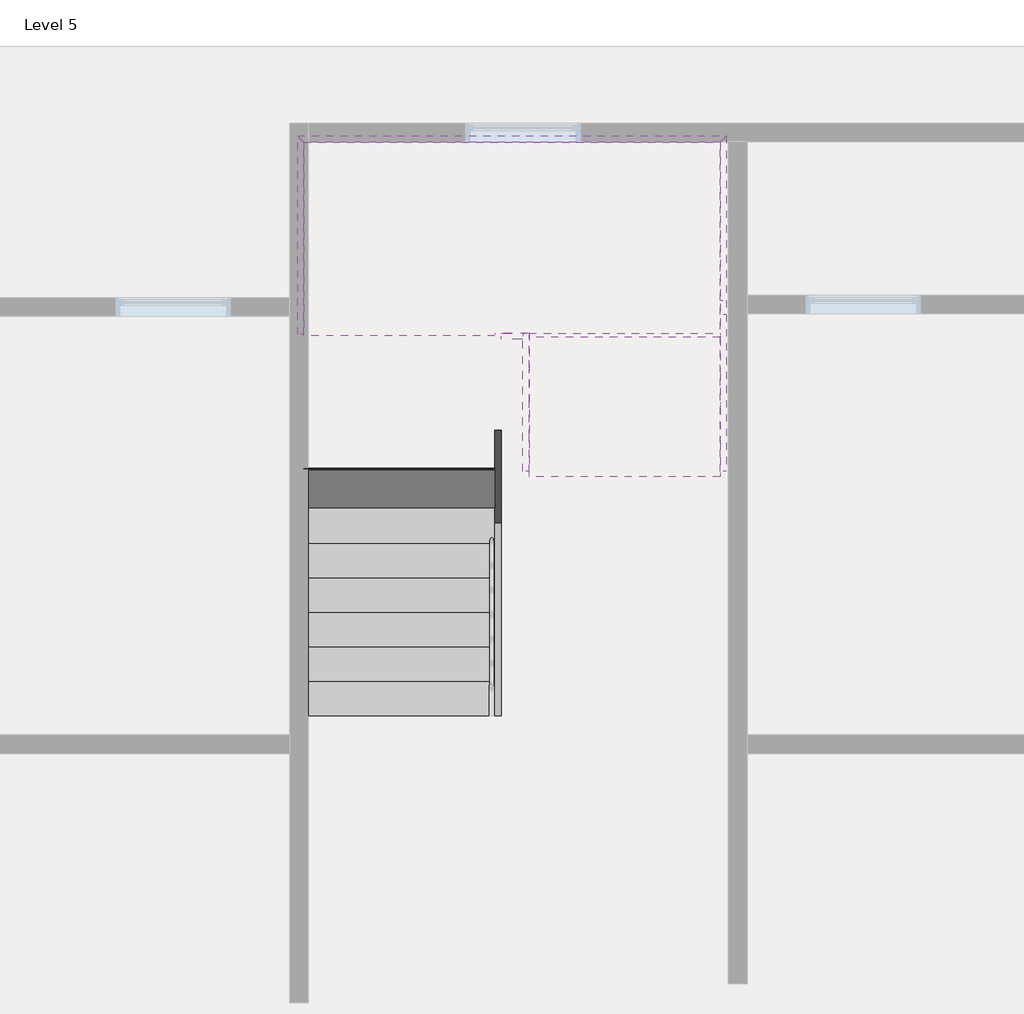
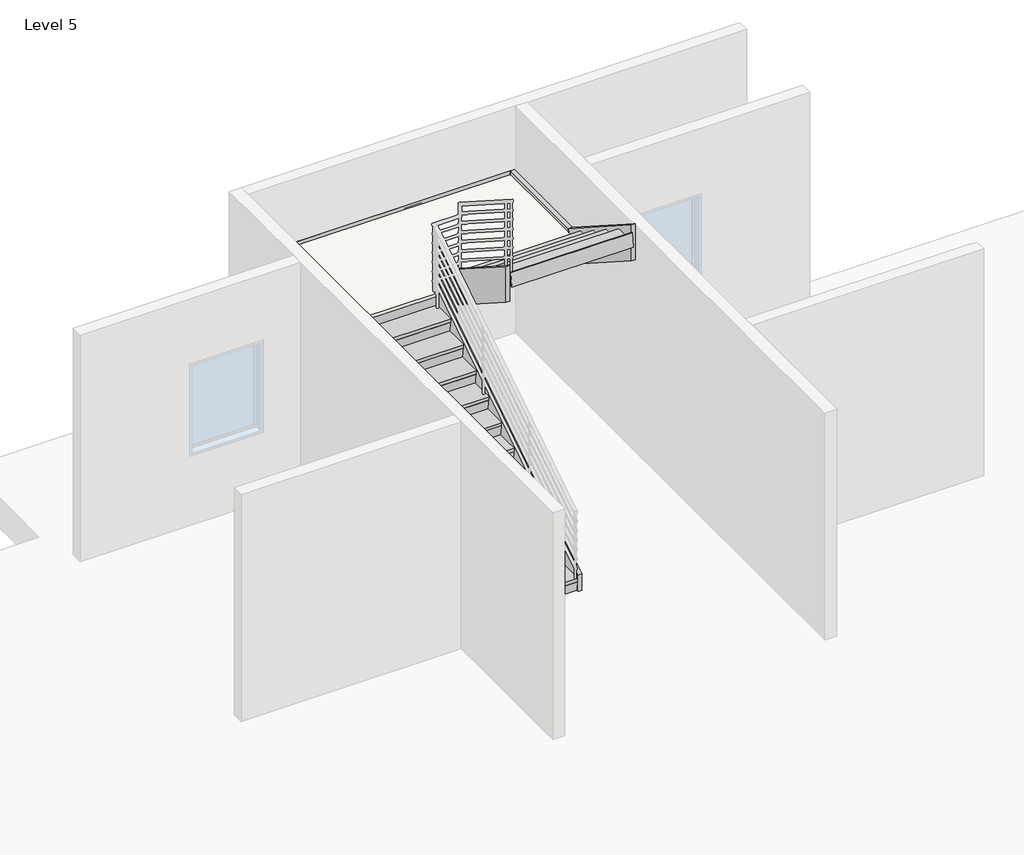
# One storey, part 7 of 7: 8 members, 2 stair flights, 1 slab.
"""IFC4 building model written with IfcOpenShell, lengths in millimetres."""

import ifcopenshell
import ifcopenshell.guid

model = None  # the IFC model being written
_history = None  # IfcOwnerHistory: only IFC2X3 demands one
_inside = {}  # id of a spatial element -> (the spatial element, [elements in it])
_under = {}  # id of a project, library or spatial element -> (it, [spatial elements below it])
_declared = {}  # id of a project -> (the project, [libraries it declares])
_typed = {}  # id of a type object -> (the type object, [elements of that type])
_made_of = {}  # id of a material, layer set ... -> (it, [elements and type objects made of it])


def new_model(schema):
    """Start an empty IFC model of exactly this schema.

    Asked for "IFC4X3", IfcOpenShell would pick the latest addendum, in which some entities
    have other attributes; the version numbers below select the first issue.
    IFC2X3 requires an IfcOwnerHistory on every rooted entity: one is made here for all.
    """
    global model, _history
    if schema == "IFC4X3":
        model = ifcopenshell.file(schema_version=(4, 3, 0, 0))
    else:
        model = ifcopenshell.file(schema=schema)
    _inside.clear()
    _under.clear()
    _declared.clear()
    _typed.clear()
    _made_of.clear()
    _history = None
    if model.schema == "IFC2X3":
        org = make("IfcOrganization", Name="unknown")
        user = make(
            "IfcPersonAndOrganization",
            ThePerson=make("IfcPerson", FamilyName="unknown"),
            TheOrganization=org,
        )
        app = make(
            "IfcApplication",
            ApplicationDeveloper=org,
            Version="unknown",
            ApplicationFullName="unknown",
            ApplicationIdentifier="unknown",
        )
        _history = make(
            "IfcOwnerHistory",
            OwningUser=user,
            OwningApplication=app,
            ChangeAction="ADDED",
            CreationDate=0,
        )
    return model


def make(cls, **values):
    """One entity of the class cls with the attributes given. An attribute that is None is left unset."""
    return model.create_entity(
        cls, **{name: value for name, value in values.items() if value is not None}
    )


def rooted(cls, **values):
    """An entity with a GlobalId (a new one), such as an element, a storey or a relation."""
    return make(cls, GlobalId=ifcopenshell.guid.new(), OwnerHistory=_history, **values)


def si_unit(unit_type, name, prefix=None):
    """IfcSIUnit, for example si_unit("LENGTHUNIT", "METRE", prefix="MILLI")."""
    return make("IfcSIUnit", UnitType=unit_type, Prefix=prefix, Name=name)


def assignment(units):
    """IfcUnitAssignment: the units of a project."""
    return None if units is None else make("IfcUnitAssignment", Units=units)


def point(xyz):
    """IfcCartesianPoint."""
    return None if xyz is None else make("IfcCartesianPoint", Coordinates=xyz)


def direction(xyz):
    """IfcDirection."""
    return None if xyz is None else make("IfcDirection", DirectionRatios=xyz)


def frame(location, z_axis=None, x_axis=None):
    """IfcAxis2Placement3D, a coordinate frame: its origin and axes. An axis left out is left unset."""
    return make(
        "IfcAxis2Placement3D",
        Location=point(location),
        Axis=direction(z_axis),
        RefDirection=direction(x_axis),
    )


def origin():
    """The frame at (0, 0, 0) with its axes left unset."""
    return frame((0.0, 0.0, 0.0))


def place(relative_to, where):
    """IfcLocalPlacement: puts the frame where relative to a parent placement (None: the world)."""
    return make(
        "IfcLocalPlacement", PlacementRelTo=relative_to, RelativePlacement=where
    )


def context(
    kind, dimensions, precision=None, world=None, true_north=None, identifier=None
):
    """IfcGeometricRepresentationContext, for example the 3D "Model" context."""
    return make(
        "IfcGeometricRepresentationContext",
        ContextIdentifier=identifier,
        ContextType=kind,
        CoordinateSpaceDimension=dimensions,
        Precision=precision,
        WorldCoordinateSystem=world,
        TrueNorth=true_north,
    )


def project(units=None, contexts=None):
    """IfcProject with its units and contexts."""
    return rooted(
        "IfcProject",
        Name="project",
        RepresentationContexts=contexts,
        UnitsInContext=assignment(units),
    )


def spatial(cls, under=None, at=None, **own):
    """A site, building, storey or space (cls), placed at a placement, below another one or the project."""
    s = rooted(cls, ObjectPlacement=at, **own)
    if under is not None:
        _under.setdefault(under.id(), (under, []))[1].append(s)
    return s


def polyline(points):
    """IfcPolyline through the points."""
    return make("IfcPolyline", Points=[point(p) for p in points])


def outline(outer, holes=None, kind="AREA"):
    """IfcArbitraryClosedProfileDef: a profile drawn as a closed curve; with holes, ...WithVoids."""
    if holes is None:
        return make("IfcArbitraryClosedProfileDef", ProfileType=kind, OuterCurve=outer)
    return make(
        "IfcArbitraryProfileDefWithVoids",
        ProfileType=kind,
        OuterCurve=outer,
        InnerCurves=holes,
    )


def extrude(swept, where, along, depth):
    """IfcExtrudedAreaSolid: the profile swept, set in the frame where, extruded along a direction by depth."""
    return make(
        "IfcExtrudedAreaSolid",
        SweptArea=swept,
        Position=where,
        ExtrudedDirection=direction(along),
        Depth=depth,
    )


def faces_of(points, faces, orient=None, outer=None):
    """IfcFace entities. A face is a list of loops; a loop is a list of indices into points, from 0.

    orient and outer hold one flag for each loop. By default every Orientation is true, the
    first loop of a face is its IfcFaceOuterBound and the others are IfcFaceBound.
    """
    made = []
    for i, loops in enumerate(faces):
        bounds = []
        for j, loop in enumerate(loops):
            is_outer = j == 0 if outer is None else outer[i][j]
            bounds.append(
                make(
                    "IfcFaceOuterBound" if is_outer else "IfcFaceBound",
                    Bound=make("IfcPolyLoop", Polygon=[points[k] for k in loop]),
                    Orientation=True if orient is None else orient[i][j],
                )
            )
        made.append(make("IfcFace", Bounds=bounds))
    return made


def faceted_brep(points, faces, orient=None, outer=None, voids=None):
    """IfcFacetedBrep: a solid bounded by flat faces; with voids (closed shells), ...WithVoids."""
    shared = [point(p) for p in points]
    hull = make("IfcClosedShell", CfsFaces=faces_of(shared, faces, orient, outer))
    if voids is None:
        return make("IfcFacetedBrep", Outer=hull)
    return make(
        "IfcFacetedBrepWithVoids",
        Outer=hull,
        Voids=[
            make(cls, CfsFaces=faces_of(shared, fs, o, b)) for cls, fs, o, b in voids
        ],
    )


def shape(context_of_items, identifier, shape_type, items):
    """IfcShapeRepresentation: the items that make up one representation, for example the "Body"."""
    return make(
        "IfcShapeRepresentation",
        ContextOfItems=context_of_items,
        RepresentationIdentifier=identifier,
        RepresentationType=shape_type,
        Items=items,
    )


def source(mapping_origin, context_of_items, identifier, shape_type, items):
    """IfcRepresentationMap: a shape defined once, which mapped items show again and again."""
    return make(
        "IfcRepresentationMap",
        MappingOrigin=mapping_origin,
        MappedRepresentation=shape(context_of_items, identifier, shape_type, items),
    )


def transform(
    local_origin,
    x_axis=None,
    y_axis=None,
    z_axis=None,
    scale=None,
    scale2=None,
    scale3=None,
    uniform=True,
):
    """IfcCartesianTransformationOperator3D, or its non-uniform kind. x_axis, y_axis, z_axis: its Axis1, 2, 3."""
    if uniform:
        return make(
            "IfcCartesianTransformationOperator3D",
            Axis1=direction(x_axis),
            Axis2=direction(y_axis),
            LocalOrigin=point(local_origin),
            Scale=scale,
            Axis3=direction(z_axis),
        )
    return make(
        "IfcCartesianTransformationOperator3DnonUniform",
        Axis1=direction(x_axis),
        Axis2=direction(y_axis),
        LocalOrigin=point(local_origin),
        Scale=scale,
        Axis3=direction(z_axis),
        Scale2=scale2,
        Scale3=scale3,
    )


def mapped(mapping_source, mapping_target):
    """IfcMappedItem: shows the shape of a source again, moved by a transform."""
    return make(
        "IfcMappedItem", MappingSource=mapping_source, MappingTarget=mapping_target
    )


def made_of(thing, what):
    """Note that an element or type object is made of a material, layer set ...; save() writes the relation."""
    if what is not None:
        _made_of.setdefault(what.id(), (what, []))[1].append(thing)
    return thing


def element(
    cls,
    number,
    at=None,
    inside=None,
    cuts=None,
    type_object=None,
    material=None,
    context=None,
    identifier="Body",
    shape_type=None,
    held_by="IfcProductDefinitionShape",
    body=None,
    shapes=None,
    **own,
):
    """One element of the class cls, such as IfcWall. Its Tag is "e" and its number.

    at: its placement. inside: the storey or other place that contains it. cuts: it is an
    opening in that element (IfcRelVoidsElement). A single representation is given by context,
    identifier, shape_type and body (its items); several are given by shapes. held_by: the class
    of the entity that holds the representations. save() writes the other relations.
    """
    e = rooted(cls, Tag="e%d" % number, ObjectPlacement=at, **own)
    if body is not None:
        shapes = [shape(context, identifier, shape_type, body)]
    if shapes is not None:
        e.Representation = make(held_by, Representations=shapes)
    if inside is not None:
        _inside.setdefault(inside.id(), (inside, []))[1].append(e)
    if cuts is not None:
        rooted(
            "IfcRelVoidsElement", RelatingBuildingElement=cuts, RelatedOpeningElement=e
        )
    if type_object is not None:
        _typed.setdefault(type_object.id(), (type_object, []))[1].append(e)
    return made_of(e, material)


def aggregate(whole, parts):
    """IfcRelAggregates: a whole, such as a stair, and the parts it consists of."""
    return rooted("IfcRelAggregates", RelatingObject=whole, RelatedObjects=parts)


def save(model, path):
    """Write the relations noted so far, then the file.

    IfcRelAggregates (storeys below a building ...), IfcRelContainedInSpatialStructure (elements
    in a storey), IfcRelDefinesByType, IfcRelAssociatesMaterial and IfcRelDeclares: one each for
    every whole, place, type object, material and project.
    """
    for whole, parts in _under.values():
        aggregate(whole, parts)
    for where, things in _inside.values():
        rooted(
            "IfcRelContainedInSpatialStructure",
            RelatedElements=things,
            RelatingStructure=where,
        )
    for kind, things in _typed.values():
        rooted("IfcRelDefinesByType", RelatedObjects=things, RelatingType=kind)
    for what, things in _made_of.values():
        rooted("IfcRelAssociatesMaterial", RelatedObjects=things, RelatingMaterial=what)
    for by, libraries in _declared.values():
        rooted("IfcRelDeclares", RelatingContext=by, RelatedDefinitions=libraries)
    model.write(path)


def non_monolithic_landing_f05efa27(model_context):
    return source(origin(), model_context, "Body", "Brep", [
        faceted_brep([(-226.7120949, 7307.4781803, 14617.6470588), (-226.7120949, 7300.3948469, 14567.6470588), (1293.2879051, 7300.3948469, 14567.6470588), (1293.2879051, 7307.4781803, 14617.6470588), (-499.4393676, 7309.7509075, 14617.6470588), (-499.4393676, 7332.4781803, 14617.6470588), (-226.7120949, 7332.4781803, 14617.6470588), (1293.2879051, 7332.4781803, 14617.6470588), (1293.2879051, 8852.4781803, 14617.6470588), (-2019.4393676, 8852.4781803, 14617.6470588), (-2019.4393676, 7309.7509075, 14617.6470588), (-226.7120949, 7332.4781803, 14567.6470588), (-499.4393676, 7332.4781803, 14567.6470588), (-499.4393676, 7316.8342409, 14567.6470588), (-2019.4393676, 7316.8342409, 14567.6470588), (-2019.4393676, 8852.4781803, 14567.6470588), (1293.2879051, 8852.4781803, 14567.6470588), (1293.2879051, 7332.4781803, 14567.6470588)], [[[0, 1, 2, 3]], [[4, 5, 6, 0, 3, 7, 8, 9, 10]], [[11, 12, 13, 14, 15, 16, 17, 2, 1]], [[5, 4, 13, 12]], [[6, 5, 12, 11]], [[0, 6, 11, 1]], [[7, 3, 2, 17]], [[8, 7, 17, 16]], [[9, 8, 16, 15]], [[10, 9, 15, 14]], [[4, 10, 14, 13]]]),
    ])


def stair_flight_50mm_tread_25mm_nosing_13mm_riser_20ac8c47(model_context):
    return source(origin(), model_context, "Body", "Brep", [
        faceted_brep([(-499.4393676, 4584.7509075, 12676.4705882), (-499.4393676, 4591.8342409, 12626.4705882), (-2019.4393676, 4591.8342409, 12626.4705882), (-2019.4393676, 4584.7509075, 12676.4705882), (-2019.4393676, 4284.7509075, 12676.4705882), (-499.4393676, 4284.7509075, 12676.4705882), (-499.4393676, 4291.8342409, 12626.4705882), (-2019.4393676, 4291.8342409, 12626.4705882)], [[[0, 1, 2, 3]], [[3, 4, 5, 0]], [[2, 1, 6, 7]], [[4, 3, 2, 7]], [[0, 5, 6, 1]], [[5, 4, 7, 6]]]),
        faceted_brep([(-499.4393676, 4291.8342409, 12626.4705882), (-499.4393676, 4309.7509075, 12500.0), (-499.4393676, 4322.3757185, 12500.0), (-499.4393676, 4304.4590518, 12626.4705882), (-2019.4393676, 4291.8342409, 12626.4705882), (-2019.4393676, 4304.4590518, 12626.4705882), (-2019.4393676, 4322.3757185, 12500.0), (-2019.4393676, 4309.7509075, 12500.0)], [[[0, 1, 2, 3]], [[4, 5, 6, 7]], [[1, 0, 4, 7]], [[2, 1, 7, 6]], [[3, 2, 6, 5]], [[0, 3, 5, 4]]]),
        faceted_brep([(-499.4393676, 4566.8342409, 12802.9411765), (-499.4393676, 4591.8342409, 12626.4705882), (-499.4393676, 4604.4590518, 12626.4705882), (-499.4393676, 4579.4590518, 12802.9411765), (-2019.4393676, 4566.8342409, 12802.9411765), (-2019.4393676, 4579.4590518, 12802.9411765), (-2019.4393676, 4604.4590518, 12626.4705882), (-2019.4393676, 4591.8342409, 12626.4705882)], [[[0, 1, 2, 3]], [[4, 5, 6, 7]], [[1, 0, 4, 7]], [[2, 1, 7, 6]], [[3, 2, 6, 5]], [[0, 3, 5, 4]]]),
        faceted_brep([(-2019.4393676, 4859.7509075, 12852.9411765), (-2019.4393676, 4559.7509075, 12852.9411765), (-499.4393676, 4559.7509075, 12852.9411765), (-499.4393676, 4859.7509075, 12852.9411765), (-2019.4393676, 4866.8342409, 12802.9411765), (-499.4393676, 4866.8342409, 12802.9411765), (-499.4393676, 4566.8342409, 12802.9411765), (-2019.4393676, 4566.8342409, 12802.9411765)], [[[0, 1, 2, 3]], [[4, 5, 6, 7]], [[1, 0, 4, 7]], [[3, 2, 6, 5]], [[3, 5, 4, 0]], [[2, 1, 7, 6]]]),
        faceted_brep([(-499.4393676, 4841.8342409, 12979.4117647), (-499.4393676, 4866.8342409, 12802.9411765), (-499.4393676, 4879.4590518, 12802.9411765), (-499.4393676, 4854.4590518, 12979.4117647), (-2019.4393676, 4841.8342409, 12979.4117647), (-2019.4393676, 4854.4590518, 12979.4117647), (-2019.4393676, 4879.4590518, 12802.9411765), (-2019.4393676, 4866.8342409, 12802.9411765)], [[[0, 1, 2, 3]], [[4, 5, 6, 7]], [[1, 0, 4, 7]], [[2, 1, 7, 6]], [[3, 2, 6, 5]], [[0, 3, 5, 4]]]),
        faceted_brep([(-2019.4393676, 5134.7509075, 13029.4117647), (-2019.4393676, 4834.7509075, 13029.4117647), (-499.4393676, 4834.7509075, 13029.4117647), (-499.4393676, 5134.7509075, 13029.4117647), (-2019.4393676, 5141.8342409, 12979.4117647), (-499.4393676, 5141.8342409, 12979.4117647), (-499.4393676, 4841.8342409, 12979.4117647), (-2019.4393676, 4841.8342409, 12979.4117647)], [[[0, 1, 2, 3]], [[4, 5, 6, 7]], [[1, 0, 4, 7]], [[3, 2, 6, 5]], [[3, 5, 4, 0]], [[2, 1, 7, 6]]]),
        faceted_brep([(-499.4393676, 5116.8342409, 13155.8823529), (-499.4393676, 5141.8342409, 12979.4117647), (-499.4393676, 5154.4590518, 12979.4117647), (-499.4393676, 5129.4590518, 13155.8823529), (-2019.4393676, 5116.8342409, 13155.8823529), (-2019.4393676, 5129.4590518, 13155.8823529), (-2019.4393676, 5154.4590518, 12979.4117647), (-2019.4393676, 5141.8342409, 12979.4117647)], [[[0, 1, 2, 3]], [[4, 5, 6, 7]], [[1, 0, 4, 7]], [[2, 1, 7, 6]], [[3, 2, 6, 5]], [[0, 3, 5, 4]]]),
        faceted_brep([(-2019.4393676, 5409.7509075, 13205.8823529), (-2019.4393676, 5109.7509075, 13205.8823529), (-499.4393676, 5109.7509075, 13205.8823529), (-499.4393676, 5409.7509075, 13205.8823529), (-2019.4393676, 5416.8342409, 13155.8823529), (-499.4393676, 5416.8342409, 13155.8823529), (-499.4393676, 5116.8342409, 13155.8823529), (-2019.4393676, 5116.8342409, 13155.8823529)], [[[0, 1, 2, 3]], [[4, 5, 6, 7]], [[1, 0, 4, 7]], [[3, 2, 6, 5]], [[3, 5, 4, 0]], [[2, 1, 7, 6]]]),
        faceted_brep([(-499.4393676, 5391.8342409, 13332.3529412), (-499.4393676, 5416.8342409, 13155.8823529), (-499.4393676, 5429.4590518, 13155.8823529), (-499.4393676, 5404.4590518, 13332.3529412), (-2019.4393676, 5391.8342409, 13332.3529412), (-2019.4393676, 5404.4590518, 13332.3529412), (-2019.4393676, 5429.4590518, 13155.8823529), (-2019.4393676, 5416.8342409, 13155.8823529)], [[[0, 1, 2, 3]], [[4, 5, 6, 7]], [[1, 0, 4, 7]], [[2, 1, 7, 6]], [[3, 2, 6, 5]], [[0, 3, 5, 4]]]),
        faceted_brep([(-2019.4393676, 5684.7509075, 13382.3529412), (-2019.4393676, 5384.7509075, 13382.3529412), (-499.4393676, 5384.7509075, 13382.3529412), (-499.4393676, 5684.7509075, 13382.3529412), (-2019.4393676, 5691.8342409, 13332.3529412), (-499.4393676, 5691.8342409, 13332.3529412), (-499.4393676, 5391.8342409, 13332.3529412), (-2019.4393676, 5391.8342409, 13332.3529412)], [[[0, 1, 2, 3]], [[4, 5, 6, 7]], [[1, 0, 4, 7]], [[3, 2, 6, 5]], [[3, 5, 4, 0]], [[2, 1, 7, 6]]]),
        faceted_brep([(-499.4393676, 5666.8342409, 13508.8235294), (-499.4393676, 5691.8342409, 13332.3529412), (-499.4393676, 5704.4590518, 13332.3529412), (-499.4393676, 5679.4590518, 13508.8235294), (-2019.4393676, 5666.8342409, 13508.8235294), (-2019.4393676, 5679.4590518, 13508.8235294), (-2019.4393676, 5704.4590518, 13332.3529412), (-2019.4393676, 5691.8342409, 13332.3529412)], [[[0, 1, 2, 3]], [[4, 5, 6, 7]], [[1, 0, 4, 7]], [[2, 1, 7, 6]], [[3, 2, 6, 5]], [[0, 3, 5, 4]]]),
        faceted_brep([(-2019.4393676, 5959.7509075, 13558.8235294), (-2019.4393676, 5659.7509075, 13558.8235294), (-499.4393676, 5659.7509075, 13558.8235294), (-499.4393676, 5959.7509075, 13558.8235294), (-2019.4393676, 5966.8342409, 13508.8235294), (-499.4393676, 5966.8342409, 13508.8235294), (-499.4393676, 5666.8342409, 13508.8235294), (-2019.4393676, 5666.8342409, 13508.8235294)], [[[0, 1, 2, 3]], [[4, 5, 6, 7]], [[1, 0, 4, 7]], [[3, 2, 6, 5]], [[3, 5, 4, 0]], [[2, 1, 7, 6]]]),
        faceted_brep([(-499.4393676, 5941.8342409, 13685.2941176), (-499.4393676, 5966.8342409, 13508.8235294), (-499.4393676, 5979.4590518, 13508.8235294), (-499.4393676, 5954.4590518, 13685.2941176), (-2019.4393676, 5941.8342409, 13685.2941176), (-2019.4393676, 5954.4590518, 13685.2941176), (-2019.4393676, 5979.4590518, 13508.8235294), (-2019.4393676, 5966.8342409, 13508.8235294)], [[[0, 1, 2, 3]], [[4, 5, 6, 7]], [[1, 0, 4, 7]], [[2, 1, 7, 6]], [[3, 2, 6, 5]], [[0, 3, 5, 4]]]),
        faceted_brep([(-2019.4393676, 6234.7509075, 13735.2941176), (-2019.4393676, 5934.7509075, 13735.2941176), (-499.4393676, 5934.7509075, 13735.2941176), (-499.4393676, 6234.7509075, 13735.2941176), (-2019.4393676, 6241.8342409, 13685.2941176), (-499.4393676, 6241.8342409, 13685.2941176), (-499.4393676, 5941.8342409, 13685.2941176), (-2019.4393676, 5941.8342409, 13685.2941176)], [[[0, 1, 2, 3]], [[4, 5, 6, 7]], [[1, 0, 4, 7]], [[3, 2, 6, 5]], [[3, 5, 4, 0]], [[2, 1, 7, 6]]]),
        faceted_brep([(-499.4393676, 6216.8342409, 13861.7647059), (-499.4393676, 6241.8342409, 13685.2941176), (-499.4393676, 6254.4590518, 13685.2941176), (-499.4393676, 6229.4590518, 13861.7647059), (-2019.4393676, 6216.8342409, 13861.7647059), (-2019.4393676, 6229.4590518, 13861.7647059), (-2019.4393676, 6254.4590518, 13685.2941176), (-2019.4393676, 6241.8342409, 13685.2941176)], [[[0, 1, 2, 3]], [[4, 5, 6, 7]], [[1, 0, 4, 7]], [[2, 1, 7, 6]], [[3, 2, 6, 5]], [[0, 3, 5, 4]]]),
        faceted_brep([(-2019.4393676, 6509.7509075, 13911.7647059), (-2019.4393676, 6209.7509075, 13911.7647059), (-499.4393676, 6209.7509075, 13911.7647059), (-499.4393676, 6509.7509075, 13911.7647059), (-2019.4393676, 6516.8342409, 13861.7647059), (-499.4393676, 6516.8342409, 13861.7647059), (-499.4393676, 6216.8342409, 13861.7647059), (-2019.4393676, 6216.8342409, 13861.7647059)], [[[0, 1, 2, 3]], [[4, 5, 6, 7]], [[1, 0, 4, 7]], [[3, 2, 6, 5]], [[3, 5, 4, 0]], [[2, 1, 7, 6]]]),
        faceted_brep([(-499.4393676, 6491.8342409, 14038.2352941), (-499.4393676, 6516.8342409, 13861.7647059), (-499.4393676, 6529.4590518, 13861.7647059), (-499.4393676, 6504.4590518, 14038.2352941), (-2019.4393676, 6491.8342409, 14038.2352941), (-2019.4393676, 6504.4590518, 14038.2352941), (-2019.4393676, 6529.4590518, 13861.7647059), (-2019.4393676, 6516.8342409, 13861.7647059)], [[[0, 1, 2, 3]], [[4, 5, 6, 7]], [[1, 0, 4, 7]], [[2, 1, 7, 6]], [[3, 2, 6, 5]], [[0, 3, 5, 4]]]),
        faceted_brep([(-2019.4393676, 6784.7509075, 14088.2352941), (-2019.4393676, 6484.7509075, 14088.2352941), (-499.4393676, 6484.7509075, 14088.2352941), (-499.4393676, 6784.7509075, 14088.2352941), (-2019.4393676, 6791.8342409, 14038.2352941), (-499.4393676, 6791.8342409, 14038.2352941), (-499.4393676, 6491.8342409, 14038.2352941), (-2019.4393676, 6491.8342409, 14038.2352941)], [[[0, 1, 2, 3]], [[4, 5, 6, 7]], [[1, 0, 4, 7]], [[3, 2, 6, 5]], [[3, 5, 4, 0]], [[2, 1, 7, 6]]]),
        faceted_brep([(-499.4393676, 6766.8342409, 14214.7058824), (-499.4393676, 6791.8342409, 14038.2352941), (-499.4393676, 6804.4590518, 14038.2352941), (-499.4393676, 6779.4590518, 14214.7058824), (-2019.4393676, 6766.8342409, 14214.7058824), (-2019.4393676, 6779.4590518, 14214.7058824), (-2019.4393676, 6804.4590518, 14038.2352941), (-2019.4393676, 6791.8342409, 14038.2352941)], [[[0, 1, 2, 3]], [[4, 5, 6, 7]], [[1, 0, 4, 7]], [[2, 1, 7, 6]], [[3, 2, 6, 5]], [[0, 3, 5, 4]]]),
        faceted_brep([(-2019.4393676, 7059.7509075, 14264.7058824), (-2019.4393676, 6759.7509075, 14264.7058824), (-499.4393676, 6759.7509075, 14264.7058824), (-499.4393676, 7059.7509075, 14264.7058824), (-2019.4393676, 7066.8342409, 14214.7058824), (-499.4393676, 7066.8342409, 14214.7058824), (-499.4393676, 6766.8342409, 14214.7058824), (-2019.4393676, 6766.8342409, 14214.7058824)], [[[0, 1, 2, 3]], [[4, 5, 6, 7]], [[1, 0, 4, 7]], [[3, 2, 6, 5]], [[3, 5, 4, 0]], [[2, 1, 7, 6]]]),
        faceted_brep([(-499.4393676, 7316.8342409, 14567.6470588), (-499.4393676, 7341.8342409, 14391.1764706), (-499.4393676, 7354.4590518, 14391.1764706), (-499.4393676, 7329.4590518, 14567.6470588), (-2019.4393676, 7316.8342409, 14567.6470588), (-2019.4393676, 7329.4590518, 14567.6470588), (-2019.4393676, 7354.4590518, 14391.1764706), (-2019.4393676, 7341.8342409, 14391.1764706)], [[[0, 1, 2, 3]], [[4, 5, 6, 7]], [[1, 0, 4, 7]], [[2, 1, 7, 6]], [[3, 2, 6, 5]], [[0, 3, 5, 4]]]),
        faceted_brep([(-499.4393676, 7041.8342409, 14391.1764706), (-499.4393676, 7066.8342409, 14214.7058824), (-499.4393676, 7079.4590518, 14214.7058824), (-499.4393676, 7054.4590518, 14391.1764706), (-2019.4393676, 7041.8342409, 14391.1764706), (-2019.4393676, 7054.4590518, 14391.1764706), (-2019.4393676, 7079.4590518, 14214.7058824), (-2019.4393676, 7066.8342409, 14214.7058824)], [[[0, 1, 2, 3]], [[4, 5, 6, 7]], [[1, 0, 4, 7]], [[2, 1, 7, 6]], [[3, 2, 6, 5]], [[0, 3, 5, 4]]]),
        faceted_brep([(-2019.4393676, 7334.7509075, 14441.1764706), (-2019.4393676, 7309.7509075, 14441.1764706), (-2019.4393676, 7034.7509075, 14441.1764706), (-499.4393676, 7034.7509075, 14441.1764706), (-499.4393676, 7334.7509075, 14441.1764706), (-2019.4393676, 7341.8342409, 14391.1764706), (-499.4393676, 7341.8342409, 14391.1764706), (-499.4393676, 7041.8342409, 14391.1764706), (-2019.4393676, 7041.8342409, 14391.1764706), (-2019.4393676, 7309.7509075, 14391.1764706)], [[[0, 1, 2, 3, 4]], [[5, 6, 7, 8, 9]], [[1, 0, 5, 9]], [[2, 1, 9, 8]], [[4, 3, 7, 6]], [[4, 6, 5, 0]], [[3, 2, 8, 7]]]),
    ])


def stair_flight_50mm_tread_25mm_nosing_13mm_riser_f085b140(model_context):
    return source(origin(), model_context, "Body", "SweptSolid", [
        extrude(outline(polyline([(7032.4781803, 14794.1176471), (7332.4781803, 14794.1176471), (7325.3948469, 14744.1176471), (7025.3948469, 14744.1176471), (7032.4781803, 14794.1176471)])), frame((-226.7120949, 0.0, 0.0), z_axis=(1.0, 0.0, 0.0), x_axis=(0.0, 1.0, 0.0)), (0.0, 0.0, 1.0), 1520.0),
        extrude(outline(polyline([(7325.3948469, 14744.1176471), (7300.3948469, 14567.6470588), (7287.770036, 14567.6470588), (7312.770036, 14744.1176471), (7325.3948469, 14744.1176471)])), frame((-226.7120949, 0.0, 0.0), z_axis=(1.0, 0.0, 0.0), x_axis=(0.0, 1.0, 0.0)), (0.0, 0.0, 1.0), 1520.0),
        extrude(outline(polyline([(7050.3948469, 14920.5882353), (7025.3948469, 14744.1176471), (7012.770036, 14744.1176471), (7037.770036, 14920.5882353), (7050.3948469, 14920.5882353)])), frame((-226.7120949, 0.0, 0.0), z_axis=(1.0, 0.0, 0.0), x_axis=(0.0, 1.0, 0.0)), (0.0, 0.0, 1.0), 1520.0),
        extrude(outline(polyline([(6757.4781803, 14970.5882353), (7057.4781803, 14970.5882353), (7050.3948469, 14920.5882353), (6750.3948469, 14920.5882353), (6757.4781803, 14970.5882353)])), frame((-226.7120949, 0.0, 0.0), z_axis=(1.0, 0.0, 0.0), x_axis=(0.0, 1.0, 0.0)), (0.0, 0.0, 1.0), 1520.0),
        extrude(outline(polyline([(6775.3948469, 15097.0588235), (6750.3948469, 14920.5882353), (6737.770036, 14920.5882353), (6762.770036, 15097.0588235), (6775.3948469, 15097.0588235)])), frame((-226.7120949, 0.0, 0.0), z_axis=(1.0, 0.0, 0.0), x_axis=(0.0, 1.0, 0.0)), (0.0, 0.0, 1.0), 1520.0),
        extrude(outline(polyline([(6482.4781803, 15147.0588235), (6782.4781803, 15147.0588235), (6775.3948469, 15097.0588235), (6475.3948469, 15097.0588235), (6482.4781803, 15147.0588235)])), frame((-226.7120949, 0.0, 0.0), z_axis=(1.0, 0.0, 0.0), x_axis=(0.0, 1.0, 0.0)), (0.0, 0.0, 1.0), 1520.0),
        extrude(outline(polyline([(6500.3948469, 15273.5294118), (6475.3948469, 15097.0588235), (6462.770036, 15097.0588235), (6487.770036, 15273.5294118), (6500.3948469, 15273.5294118)])), frame((-226.7120949, 0.0, 0.0), z_axis=(1.0, 0.0, 0.0), x_axis=(0.0, 1.0, 0.0)), (0.0, 0.0, 1.0), 1520.0),
        extrude(outline(polyline([(6225.3948469, 15450.0), (6200.3948469, 15273.5294118), (6187.770036, 15273.5294118), (6212.770036, 15450.0), (6225.3948469, 15450.0)])), frame((-226.7120949, 0.0, 0.0), z_axis=(1.0, 0.0, 0.0), x_axis=(0.0, 1.0, 0.0)), (0.0, 0.0, 1.0), 1520.0),
        extrude(outline(polyline([(6207.4781803, 15323.5294118), (6507.4781803, 15323.5294118), (6500.3948469, 15273.5294118), (6200.3948469, 15273.5294118), (6207.4781803, 15323.5294118)])), frame((-226.7120949, 0.0, 0.0), z_axis=(1.0, 0.0, 0.0), x_axis=(0.0, 1.0, 0.0)), (0.0, 0.0, 1.0), 1520.0),
    ])


model = new_model("IFC4")

# Units and contexts
model_context = context("Model", 3, world=origin())
ifc_project = project(units=[si_unit("LENGTHUNIT", "METRE", prefix="MILLI")], contexts=[model_context])

# Site, building, storey
site = spatial("IfcSite", under=ifc_project)
building = spatial("IfcBuilding", under=site)
storey = spatial("IfcBuildingStorey", under=building, Name="Level 5", Elevation=12500.0)

# Members
placement = place(None, origin())
element("IfcMember", 1, ObjectType="Stringer - 50mm Width", at=placement, inside=storey, context=model_context, shape_type="SweptSolid", body=[
    extrude(outline(polyline([(4284.7509075, 12500.0), (4284.7509075, 12715.9811749), (7322.0354678, 14665.0407858), (7439.3399977, 14265.0407858), (4688.8181065, 12500.0), (4284.7509075, 12500.0)])), frame((-2069.4393676, 0.0, 0.0), z_axis=(1.0, 0.0, 0.0), x_axis=(0.0, 1.0, 0.0)), (0.0, 0.0, 1.0), 50.0),
])
element("IfcMember", 2, ObjectType="Stringer - 50mm Width", at=placement, inside=storey, context=model_context, shape_type="SweptSolid", body=[
    extrude(outline(polyline([(4284.7509075, 12500.0), (4284.7509075, 12715.9811749), (7322.0354678, 14665.0407858), (7332.4781803, 14665.0407858), (7332.4781803, 14196.4663575), (4688.8181065, 12500.0), (4284.7509075, 12500.0)])), frame((-499.4393676, 0.0, 0.0), z_axis=(1.0, 0.0, 0.0), x_axis=(0.0, 1.0, 0.0)), (0.0, 0.0, 1.0), 50.0),
])
element("IfcMember", 3, ObjectType="Stringer - 50mm Width", at=placement, inside=storey, context=model_context, shape_type="SweptSolid", body=[
    extrude(outline(polyline([(7595.19362, 14665.0407858), (7477.8890902, 14265.0407858), (6232.4781803, 15064.2349525), (6232.4781803, 15539.5105867), (7595.19362, 14665.0407858)])), frame((1293.2879051, 0.0, 0.0), z_axis=(1.0, 0.0, 0.0), x_axis=(0.0, 1.0, 0.0)), (0.0, 0.0, 1.0), 50.0),
])
element("IfcMember", 4, ObjectType="Stringer - 50mm Width", at=placement, inside=storey, context=model_context, shape_type="SweptSolid", body=[
    extrude(outline(polyline([(7332.4781803, 14833.6282338), (7332.4781803, 14358.3525996), (6232.4781803, 15064.2349525), (6232.4781803, 15539.5105867), (7332.4781803, 14833.6282338)])), frame((-276.7120949, 0.0, 0.0), z_axis=(1.0, 0.0, 0.0), x_axis=(0.0, 1.0, 0.0)), (0.0, 0.0, 1.0), 50.0),
])
element("IfcMember", 5, ObjectType="Stringer - 50mm Width", at=placement, inside=storey, context=model_context, shape_type="Brep", body=[
    faceted_brep([(1293.2879051, 7595.19362, 14665.0407858), (1343.2879051, 7595.19362, 14665.0407858), (1343.2879051, 8902.4781803, 14665.0407858), (1293.2879051, 8852.4781803, 14665.0407858), (1293.2879051, 7477.8890902, 14265.0407858), (1293.2879051, 8852.4781803, 14265.0407858), (1343.2879051, 7477.8890902, 14265.0407858), (1343.2879051, 8902.4781803, 14265.0407858)], [[[0, 1, 2, 3]], [[4, 0, 3, 5]], [[6, 4, 5, 7]], [[1, 6, 7, 2]], [[1, 0, 4, 6]], [[2, 7, 5, 3]]]),
])
element("IfcMember", 6, ObjectType="Stringer - 50mm Width", at=placement, inside=storey, context=model_context, shape_type="SweptSolid", body=[
    extrude(outline(polyline([(1343.2879051, 8902.4781803), (1293.2879051, 8852.4781803), (-2019.4393676, 8852.4781803), (-2069.4393676, 8902.4781803), (1343.2879051, 8902.4781803)])), frame((0.0, 0.0, 14265.0407858), z_axis=(0.0, 0.0, 1.0), x_axis=(1.0, 0.0, 0.0)), (0.0, 0.0, 1.0), 400.0),
])
element("IfcMember", 7, ObjectType="Stringer - 50mm Width", at=placement, inside=storey, context=model_context, shape_type="Brep", body=[
    faceted_brep([(-2019.4393676, 8852.4781803, 14665.0407858), (-2069.4393676, 8902.4781803, 14665.0407858), (-2069.4393676, 7322.0354678, 14665.0407858), (-2019.4393676, 7322.0354678, 14665.0407858), (-2019.4393676, 8852.4781803, 14265.0407858), (-2019.4393676, 7439.3399977, 14265.0407858), (-2069.4393676, 8902.4781803, 14265.0407858), (-2069.4393676, 7439.3399977, 14265.0407858)], [[[0, 1, 2, 3]], [[4, 0, 3, 5]], [[6, 4, 5, 7]], [[1, 6, 7, 2]], [[1, 0, 4, 6]], [[2, 7, 5, 3]]]),
])
element("IfcMember", 8, ObjectType="Stringer - 50mm Width", at=placement, inside=storey, context=model_context, shape_type="SweptSolid", body=[
    extrude(outline(polyline([(-449.4393676, 7282.4781803), (-449.4393676, 7332.4781803), (-276.7120949, 7332.4781803), (-276.7120949, 7282.4781803), (-449.4393676, 7282.4781803)])), frame((0.0, 0.0, 14265.0407858), z_axis=(0.0, 0.0, 1.0), x_axis=(1.0, 0.0, 0.0)), (0.0, 0.0, 1.0), 400.0),
])

# Slab
non_monolithic_landing_shape = non_monolithic_landing_f05efa27(model_context)
element("IfcSlab", 9, ObjectType="Non-Monolithic Landing", at=placement, inside=storey, context=model_context, shape_type="MappedRepresentation", body=[
    mapped(non_monolithic_landing_shape, transform((0.0, 0.0, 0.0), x_axis=(1.0, 0.0, 0.0), y_axis=(0.0, 1.0, 0.0), z_axis=(0.0, 0.0, 1.0))),
])

# Stair flights
stair_flight_50mm_tread_25mm_nosing_13mm_riser_shape = stair_flight_50mm_tread_25mm_nosing_13mm_riser_20ac8c47(model_context)
element("IfcStairFlight", 10, ObjectType="50mm Tread 25mm Nosing 13mm Riser", at=placement, inside=storey, context=model_context, shape_type="MappedRepresentation", body=[
    mapped(stair_flight_50mm_tread_25mm_nosing_13mm_riser_shape, transform((0.0, 0.0, 0.0), x_axis=(1.0, 0.0, 0.0), y_axis=(0.0, 1.0, 0.0), z_axis=(0.0, 0.0, 1.0))),
])
stair_flight_50mm_tread_25mm_nosing_13mm_riser_2_shape = stair_flight_50mm_tread_25mm_nosing_13mm_riser_f085b140(model_context)
element("IfcStairFlight", 11, ObjectType="50mm Tread 25mm Nosing 13mm Riser", at=placement, inside=storey, context=model_context, shape_type="MappedRepresentation", body=[
    mapped(stair_flight_50mm_tread_25mm_nosing_13mm_riser_2_shape, transform((0.0, 0.0, 0.0), x_axis=(1.0, 0.0, 0.0), y_axis=(0.0, 1.0, 0.0), z_axis=(0.0, 0.0, 1.0))),
])

save(model, "model.ifc")

# Revit data of these elements
# Elements 1, 2, 3, 4, 5, 6, 7, 8 (IfcMember, "Stringer - 50mm Width")
#   Phase Created = New Construction
# Element 9 (IfcSlab, "Non-Monolithic Landing")
#   Phase Created = New Construction
# Elements 10, 11 (IfcStairFlight, "50mm Tread 25mm Nosing 13mm Riser")
#   Phase Created = New Construction
